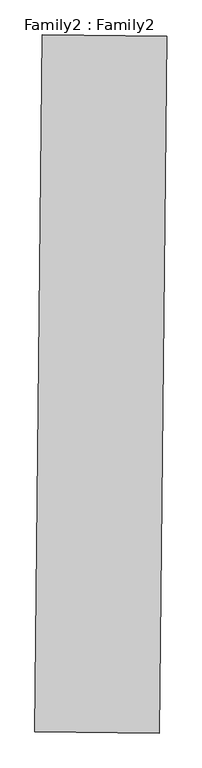
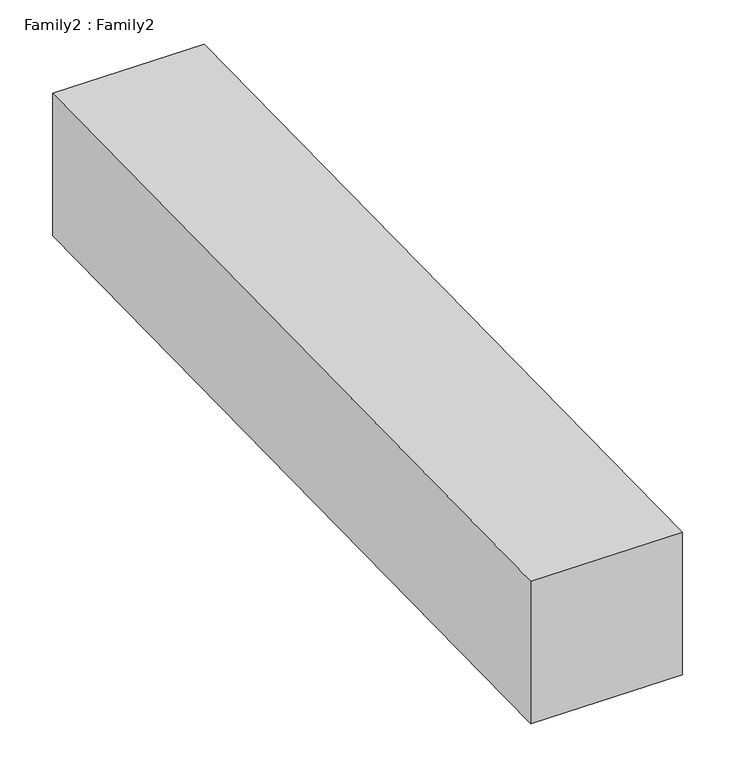
"""IFC4 building model written with IfcOpenShell, lengths in millimetres: proxy geometry, Family2 : Family2."""

from ifc_helpers import new_model, si_unit, origin, place, context, project, spatial, faceted_brep, source, transform, mapped, element, save


def family2_family2_53b3ea5e(model_context):
    return source(origin(), model_context, "Body", "Brep", [
        faceted_brep([(-3949.4952094, -6634.0997486, 1.0945136), (-3949.4952094, -6634.0997486, 201.0945136), (-3937.3475851, -5513.500374, 202.060409), (-3937.3475851, -5513.500374, 2.060409), (-3749.5040194, -6635.9769613, 201.0945136), (-3737.3563951, -5515.3775867, 202.060409), (-3749.5040194, -6635.9769613, 1.0945136), (-3737.3563951, -5515.3775867, 2.060409)], [[[0, 1, 2, 3]], [[1, 4, 5, 2]], [[4, 6, 7, 5]], [[6, 0, 3, 7]], [[3, 2, 5, 7]], [[0, 6, 4, 1]]]),
    ])


if __name__ == "__main__":
    model = new_model("IFC4")
    model_context = context("Model", 3, world=origin())
    ifc_project = project(units=[si_unit("LENGTHUNIT", "METRE", prefix="MILLI")], contexts=[model_context])
    site = spatial("IfcSite", under=ifc_project)
    building = spatial("IfcBuilding", under=site)
    placement = place(None, origin())
    family2_family2_shape = family2_family2_53b3ea5e(model_context)
    element("IfcBuildingElementProxy", 1, Name="Family2 : Family2", ObjectType="Family2 : Family2", at=placement, inside=building, context=model_context, shape_type="MappedRepresentation", body=[
        mapped(family2_family2_shape, transform((0.0, 0.0, 0.0), x_axis=(1.0, 0.0, 0.0), y_axis=(0.0, 1.0, 0.0), z_axis=(0.0, 0.0, 1.0))),
    ])
    save(model, "model.ifc")

# Revit data of these elements
# Type "Family2 : Family2"
#   Default Elevation = 0
